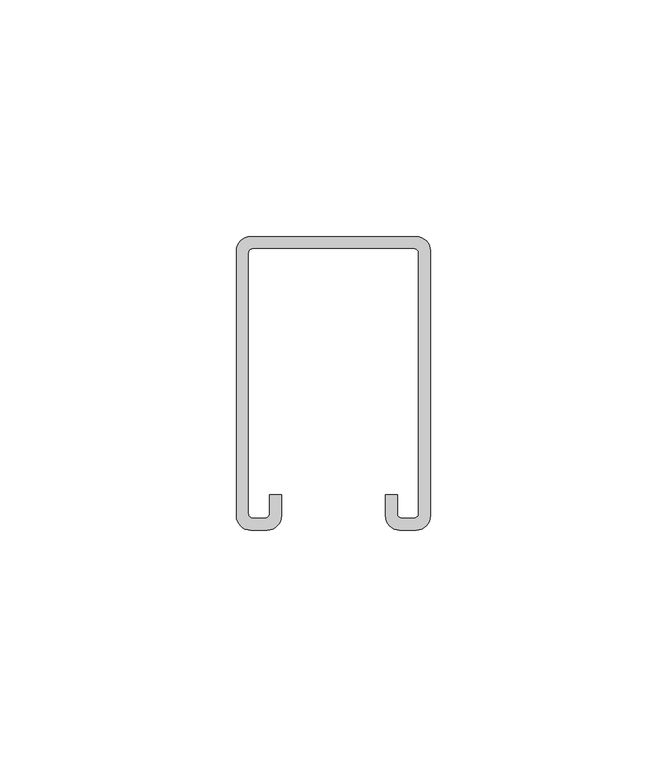
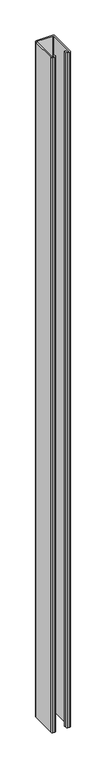
"""IFC4 building model written with IfcOpenShell, lengths in millimetres: proxy geometry, TN_Профиль монтажный : Профиль монтажный 41x62x2,5-3000."""

import ifcopenshell
import ifcopenshell.guid

model = None  # the IFC model being written
_history = None  # IfcOwnerHistory: only IFC2X3 demands one
_inside = {}  # id of a spatial element -> (the spatial element, [elements in it])
_under = {}  # id of a project, library or spatial element -> (it, [spatial elements below it])
_declared = {}  # id of a project -> (the project, [libraries it declares])
_typed = {}  # id of a type object -> (the type object, [elements of that type])
_made_of = {}  # id of a material, layer set ... -> (it, [elements and type objects made of it])


def new_model(schema):
    """Start an empty IFC model of exactly this schema.

    Asked for "IFC4X3", IfcOpenShell would pick the latest addendum, in which some entities
    have other attributes; the version numbers below select the first issue.
    IFC2X3 requires an IfcOwnerHistory on every rooted entity: one is made here for all.
    """
    global model, _history
    if schema == "IFC4X3":
        model = ifcopenshell.file(schema_version=(4, 3, 0, 0))
    else:
        model = ifcopenshell.file(schema=schema)
    _inside.clear()
    _under.clear()
    _declared.clear()
    _typed.clear()
    _made_of.clear()
    _history = None
    if model.schema == "IFC2X3":
        org = make("IfcOrganization", Name="unknown")
        user = make(
            "IfcPersonAndOrganization",
            ThePerson=make("IfcPerson", FamilyName="unknown"),
            TheOrganization=org,
        )
        app = make(
            "IfcApplication",
            ApplicationDeveloper=org,
            Version="unknown",
            ApplicationFullName="unknown",
            ApplicationIdentifier="unknown",
        )
        _history = make(
            "IfcOwnerHistory",
            OwningUser=user,
            OwningApplication=app,
            ChangeAction="ADDED",
            CreationDate=0,
        )
    return model


def make(cls, **values):
    """One entity of the class cls with the attributes given. An attribute that is None is left unset."""
    return model.create_entity(
        cls, **{name: value for name, value in values.items() if value is not None}
    )


def rooted(cls, **values):
    """An entity with a GlobalId (a new one), such as an element, a storey or a relation."""
    return make(cls, GlobalId=ifcopenshell.guid.new(), OwnerHistory=_history, **values)


def si_unit(unit_type, name, prefix=None):
    """IfcSIUnit, for example si_unit("LENGTHUNIT", "METRE", prefix="MILLI")."""
    return make("IfcSIUnit", UnitType=unit_type, Prefix=prefix, Name=name)


def assignment(units):
    """IfcUnitAssignment: the units of a project."""
    return None if units is None else make("IfcUnitAssignment", Units=units)


def point(xyz):
    """IfcCartesianPoint."""
    return None if xyz is None else make("IfcCartesianPoint", Coordinates=xyz)


def direction(xyz):
    """IfcDirection."""
    return None if xyz is None else make("IfcDirection", DirectionRatios=xyz)


def frame(location, z_axis=None, x_axis=None):
    """IfcAxis2Placement3D, a coordinate frame: its origin and axes. An axis left out is left unset."""
    return make(
        "IfcAxis2Placement3D",
        Location=point(location),
        Axis=direction(z_axis),
        RefDirection=direction(x_axis),
    )


def frame_2d(location, x_axis=None):
    """IfcAxis2Placement2D, a coordinate frame in the plane: its origin and x axis."""
    return make(
        "IfcAxis2Placement2D", Location=point(location), RefDirection=direction(x_axis)
    )


def origin():
    """The frame at (0, 0, 0) with its axes left unset."""
    return frame((0.0, 0.0, 0.0))


def origin_with_axes():
    """The frame at (0, 0, 0) with the z axis (0, 0, 1) and the x axis (1, 0, 0) written out."""
    return frame((0.0, 0.0, 0.0), z_axis=(0.0, 0.0, 1.0), x_axis=(1.0, 0.0, 0.0))


def place(relative_to, where):
    """IfcLocalPlacement: puts the frame where relative to a parent placement (None: the world)."""
    return make(
        "IfcLocalPlacement", PlacementRelTo=relative_to, RelativePlacement=where
    )


def context(
    kind, dimensions, precision=None, world=None, true_north=None, identifier=None
):
    """IfcGeometricRepresentationContext, for example the 3D "Model" context."""
    return make(
        "IfcGeometricRepresentationContext",
        ContextIdentifier=identifier,
        ContextType=kind,
        CoordinateSpaceDimension=dimensions,
        Precision=precision,
        WorldCoordinateSystem=world,
        TrueNorth=true_north,
    )


def project(units=None, contexts=None):
    """IfcProject with its units and contexts."""
    return rooted(
        "IfcProject",
        Name="project",
        RepresentationContexts=contexts,
        UnitsInContext=assignment(units),
    )


def spatial(cls, under=None, at=None, **own):
    """A site, building, storey or space (cls), placed at a placement, below another one or the project."""
    s = rooted(cls, ObjectPlacement=at, **own)
    if under is not None:
        _under.setdefault(under.id(), (under, []))[1].append(s)
    return s


def polyline(points):
    """IfcPolyline through the points."""
    return make("IfcPolyline", Points=[point(p) for p in points])


def circle_curve(where, radius):
    """IfcCircle in the frame where."""
    return make("IfcCircle", Position=where, Radius=radius)


def trimmed(basis, trim1, trim2, sense, master):
    """IfcTrimmedCurve: the piece of a basis curve between two trims."""
    return make(
        "IfcTrimmedCurve",
        BasisCurve=basis,
        Trim1=trim1,
        Trim2=trim2,
        SenseAgreement=sense,
        MasterRepresentation=master,
    )


def segment(curve, same_sense, transition):
    """IfcCompositeCurveSegment."""
    return make(
        "IfcCompositeCurveSegment",
        Transition=transition,
        SameSense=same_sense,
        ParentCurve=curve,
    )


def composite_curve(segments, self_intersect=None):
    """IfcCompositeCurve: segments joined end to end."""
    return make("IfcCompositeCurve", Segments=segments, SelfIntersect=self_intersect)


def outline(outer, holes=None, kind="AREA"):
    """IfcArbitraryClosedProfileDef: a profile drawn as a closed curve; with holes, ...WithVoids."""
    if holes is None:
        return make("IfcArbitraryClosedProfileDef", ProfileType=kind, OuterCurve=outer)
    return make(
        "IfcArbitraryProfileDefWithVoids",
        ProfileType=kind,
        OuterCurve=outer,
        InnerCurves=holes,
    )


def extrude(swept, where, along, depth):
    """IfcExtrudedAreaSolid: the profile swept, set in the frame where, extruded along a direction by depth."""
    return make(
        "IfcExtrudedAreaSolid",
        SweptArea=swept,
        Position=where,
        ExtrudedDirection=direction(along),
        Depth=depth,
    )


def shape(context_of_items, identifier, shape_type, items):
    """IfcShapeRepresentation: the items that make up one representation, for example the "Body"."""
    return make(
        "IfcShapeRepresentation",
        ContextOfItems=context_of_items,
        RepresentationIdentifier=identifier,
        RepresentationType=shape_type,
        Items=items,
    )


def source(mapping_origin, context_of_items, identifier, shape_type, items):
    """IfcRepresentationMap: a shape defined once, which mapped items show again and again."""
    return make(
        "IfcRepresentationMap",
        MappingOrigin=mapping_origin,
        MappedRepresentation=shape(context_of_items, identifier, shape_type, items),
    )


def transform(
    local_origin,
    x_axis=None,
    y_axis=None,
    z_axis=None,
    scale=None,
    scale2=None,
    scale3=None,
    uniform=True,
):
    """IfcCartesianTransformationOperator3D, or its non-uniform kind. x_axis, y_axis, z_axis: its Axis1, 2, 3."""
    if uniform:
        return make(
            "IfcCartesianTransformationOperator3D",
            Axis1=direction(x_axis),
            Axis2=direction(y_axis),
            LocalOrigin=point(local_origin),
            Scale=scale,
            Axis3=direction(z_axis),
        )
    return make(
        "IfcCartesianTransformationOperator3DnonUniform",
        Axis1=direction(x_axis),
        Axis2=direction(y_axis),
        LocalOrigin=point(local_origin),
        Scale=scale,
        Axis3=direction(z_axis),
        Scale2=scale2,
        Scale3=scale3,
    )


def mapped(mapping_source, mapping_target):
    """IfcMappedItem: shows the shape of a source again, moved by a transform."""
    return make(
        "IfcMappedItem", MappingSource=mapping_source, MappingTarget=mapping_target
    )


def made_of(thing, what):
    """Note that an element or type object is made of a material, layer set ...; save() writes the relation."""
    if what is not None:
        _made_of.setdefault(what.id(), (what, []))[1].append(thing)
    return thing


def element(
    cls,
    number,
    at=None,
    inside=None,
    cuts=None,
    type_object=None,
    material=None,
    context=None,
    identifier="Body",
    shape_type=None,
    held_by="IfcProductDefinitionShape",
    body=None,
    shapes=None,
    **own,
):
    """One element of the class cls, such as IfcWall. Its Tag is "e" and its number.

    at: its placement. inside: the storey or other place that contains it. cuts: it is an
    opening in that element (IfcRelVoidsElement). A single representation is given by context,
    identifier, shape_type and body (its items); several are given by shapes. held_by: the class
    of the entity that holds the representations. save() writes the other relations.
    """
    e = rooted(cls, Tag="e%d" % number, ObjectPlacement=at, **own)
    if body is not None:
        shapes = [shape(context, identifier, shape_type, body)]
    if shapes is not None:
        e.Representation = make(held_by, Representations=shapes)
    if inside is not None:
        _inside.setdefault(inside.id(), (inside, []))[1].append(e)
    if cuts is not None:
        rooted(
            "IfcRelVoidsElement", RelatingBuildingElement=cuts, RelatedOpeningElement=e
        )
    if type_object is not None:
        _typed.setdefault(type_object.id(), (type_object, []))[1].append(e)
    return made_of(e, material)


def aggregate(whole, parts):
    """IfcRelAggregates: a whole, such as a stair, and the parts it consists of."""
    return rooted("IfcRelAggregates", RelatingObject=whole, RelatedObjects=parts)


def save(model, path):
    """Write the relations noted so far, then the file.

    IfcRelAggregates (storeys below a building ...), IfcRelContainedInSpatialStructure (elements
    in a storey), IfcRelDefinesByType, IfcRelAssociatesMaterial and IfcRelDeclares: one each for
    every whole, place, type object, material and project.
    """
    for whole, parts in _under.values():
        aggregate(whole, parts)
    for where, things in _inside.values():
        rooted(
            "IfcRelContainedInSpatialStructure",
            RelatedElements=things,
            RelatingStructure=where,
        )
    for kind, things in _typed.values():
        rooted("IfcRelDefinesByType", RelatedObjects=things, RelatingType=kind)
    for what, things in _made_of.values():
        rooted("IfcRelAssociatesMaterial", RelatedObjects=things, RelatingMaterial=what)
    for by, libraries in _declared.values():
        rooted("IfcRelDeclares", RelatingContext=by, RelatedDefinitions=libraries)
    model.write(path)


def generic_models_83125b11(model_context):
    return source(origin(), model_context, "Body", "SweptSolid", [
        extrude(outline(composite_curve([segment(trimmed(circle_curve(frame_2d((-17.5, -3.0)), 3.0), [point((-20.5, -3.0))], [point((-17.5, 0.0))], False, "CARTESIAN"), True, "CONTINUOUS"), segment(polyline([(-17.5, 0.0), (17.5, 0.0)]), True, "CONTINUOUS"), segment(trimmed(circle_curve(frame_2d((17.5, -3.0)), 3.0), [point((17.5, 0.0))], [point((20.5, -3.0))], False, "CARTESIAN"), True, "CONTINUOUS"), segment(polyline([(20.5, -3.0), (20.5, -59.0)]), True, "CONTINUOUS"), segment(trimmed(circle_curve(frame_2d((17.5, -59.0)), 3.0), [point((20.5, -59.0))], [point((17.5, -62.0))], False, "CARTESIAN"), True, "CONTINUOUS"), segment(polyline([(17.5, -62.0), (14.0, -62.0)]), True, "CONTINUOUS"), segment(trimmed(circle_curve(frame_2d((14.0, -59.0)), 3.0), [point((14.0, -62.0))], [point((11.0, -59.0))], False, "CARTESIAN"), True, "CONTINUOUS"), segment(polyline([(11.0, -59.0), (11.0, -54.5), (13.5, -54.5), (13.5, -58.5)]), True, "CONTINUOUS"), segment(trimmed(circle_curve(frame_2d((14.5, -58.5)), 1.0), [point((13.5, -58.5))], [point((14.5, -59.5))], True, "CARTESIAN"), True, "CONTINUOUS"), segment(polyline([(14.5, -59.5), (17.0, -59.5)]), True, "CONTINUOUS"), segment(trimmed(circle_curve(frame_2d((17.0, -58.5)), 1.0), [point((17.0, -59.5))], [point((18.0, -58.5))], True, "CARTESIAN"), True, "CONTINUOUS"), segment(polyline([(18.0, -58.5), (18.0, -3.5)]), True, "CONTINUOUS"), segment(trimmed(circle_curve(frame_2d((17.0, -3.5)), 1.0), [point((18.0, -3.5))], [point((17.0, -2.5))], True, "CARTESIAN"), True, "CONTINUOUS"), segment(polyline([(17.0, -2.5), (-17.0, -2.5)]), True, "CONTINUOUS"), segment(trimmed(circle_curve(frame_2d((-17.0, -3.5)), 1.0), [point((-17.0, -2.5))], [point((-18.0, -3.5))], True, "CARTESIAN"), True, "CONTINUOUS"), segment(polyline([(-18.0, -3.5), (-18.0, -58.5)]), True, "CONTINUOUS"), segment(trimmed(circle_curve(frame_2d((-17.0, -58.5)), 1.0), [point((-18.0, -58.5))], [point((-17.0, -59.5))], True, "CARTESIAN"), True, "CONTINUOUS"), segment(polyline([(-17.0, -59.5), (-14.5, -59.5)]), True, "CONTINUOUS"), segment(trimmed(circle_curve(frame_2d((-14.5, -58.5)), 1.0), [point((-14.5, -59.5))], [point((-13.5, -58.5))], True, "CARTESIAN"), True, "CONTINUOUS"), segment(polyline([(-13.5, -58.5), (-13.5, -54.5), (-11.0, -54.5), (-11.0, -58.9588961)]), True, "CONTINUOUS"), segment(trimmed(circle_curve(frame_2d((-14.0411039, -58.9588961)), 3.0411039), [point((-11.0, -58.9588961))], [point((-14.0411039, -62.0))], False, "CARTESIAN"), True, "CONTINUOUS"), segment(polyline([(-14.0411039, -62.0), (-17.5, -62.0)]), True, "CONTINUOUS"), segment(trimmed(circle_curve(frame_2d((-17.5, -59.0)), 3.0), [point((-17.5, -62.0))], [point((-20.5, -59.0))], False, "CARTESIAN"), True, "CONTINUOUS"), segment(polyline([(-20.5, -59.0), (-20.5, -3.0)]), True, "CONTINUOUS")], self_intersect=False)), origin_with_axes(), (0.0, 0.0, 1.0), 1500.0),
    ])


if __name__ == "__main__":
    model = new_model("IFC4")
    model_context = context("Model", 3, world=origin())
    ifc_project = project(units=[si_unit("LENGTHUNIT", "METRE", prefix="MILLI")], contexts=[model_context])
    site = spatial("IfcSite", under=ifc_project)
    building = spatial("IfcBuilding", under=site)
    placement = place(None, origin())
    generic_models_shape = generic_models_83125b11(model_context)
    element("IfcBuildingElementProxy", 1, Name="TN_Профиль монтажный : Профиль монтажный 41x62x2,5-3000", ObjectType="TN_Профиль монтажный : Профиль монтажный 41x62x2,5-3000", at=placement, inside=building, context=model_context, shape_type="MappedRepresentation", body=[
        mapped(generic_models_shape, transform((0.0, 0.0, 0.0), x_axis=(1.0, 0.0, 0.0), y_axis=(0.0, 1.0, 0.0), z_axis=(0.0, 0.0, 1.0))),
    ])
    save(model, "model.ifc")

# Revit data of these elements
# Type "TN_Профиль монтажный : Профиль монтажный 41x62x2,5-3000"
#   Description = "Профиль монтажный – траверса С-образной формы предназначен для горизонтального и вертикального монтажа тяжелых инженерных систем, оборудования систем вентиляции и кондиционирования, установок электроснабжения, элементов трубопроводов, также для изготовления стенных консолей пристенного монтажа, рам оснований различного типа под оборудование. Возможно замещение на основе сконструированных модулей серийных опор ГОСТ для раскрепления технологических трубопроводов. Рекомендуется для применения в сухих, влажных помещениях и на открытом воздухе."
#   Manufacturer = "ТехноНИКОЛЬ"
#   Model = "Комплектующие к опорам"
#   URL = "https://nav.tn.ru/knowledge-base/polimernye-membrany/opory-pod-oborudovanie-na-ploskoy-krovle/?sphrase_id=266812"
#   ADSK_Обозначение = "ТехноНИКОЛЬ"
#   ADSK_Наименование краткое = "П41x62x2,5"
#   ADSK_Наименование = "Профиль монтажный 41x62x2,5-3000"
#   ADSK_Масса_Текст = ""
#   ADSK_Марка = "П41x62x2,5"
#   ADSK_Код изделия = "660817"
#   ADSK_Завод-изготовитель = "ТехноНИКОЛЬ"
#   ADSK_Единица измерения = "п.м."
#   ADSK_Группирование = "Комплектующие к опорам"
#   ADSK_URL страницы изделия = "https://nav.tn.ru/knowledge-base/polimernye-membrany/opory-pod-oborudovanie-na-ploskoy-krovle/?sphrase_id=266812"
#   ADSK_URL документации изделия = ""
#   Размер_Длина_Вводимая [instance default] = 1000 mm
#   ADSK_Размер_Длина [instance default] = 1000 mm
#   ADSK_Количество [instance default] = 1
#   Тип профиля = 1
#   Профиль монтажный 41х41x2,0 = no
#   Профиль монтажный 41x62x2,5 = yes
#   Профиль монтажный 41x124x2,5 = no
#   ADSK_Материал = TN_СтальГальванизированная_Серый
#   Default Elevation = 0
# Element 1 (IfcBuildingElementProxy, "TN_Профиль монтажный : Профиль монтажный 41x62x2,5-3000")
#   Размер_Длина_Вводимая = 1500 mm
#   ADSK_Размер_Длина = 1500 mm
#   ADSK_Количество = 1.5
#   Materials on its faces: "TN_СтальГальванизированная_Серый"
# Materials
#   "TN_СтальГальванизированная_Серый": class "Типовые", colour RGB 206 210 213, transparency 0, Cost = 0
